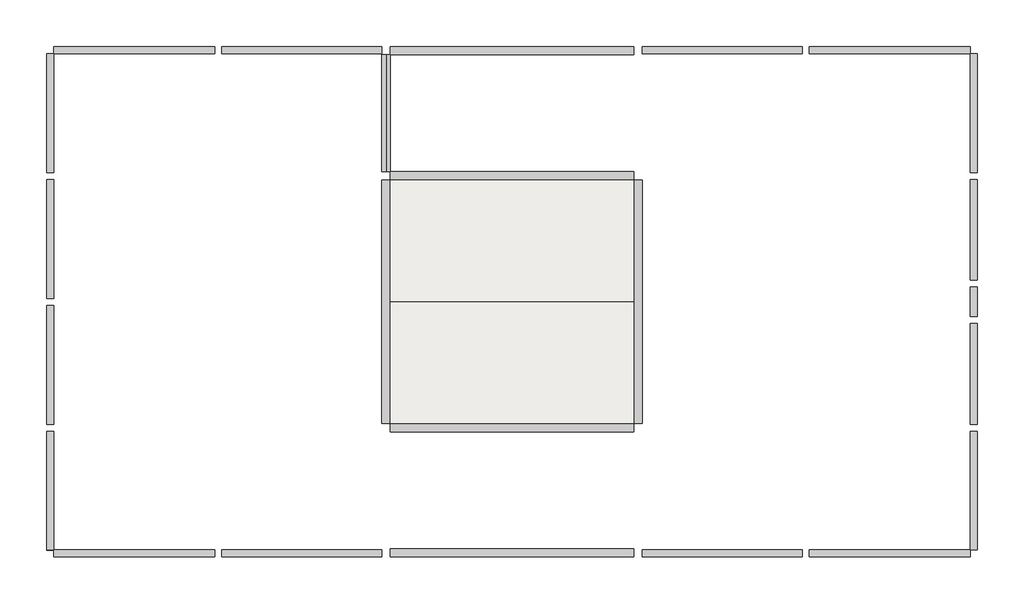
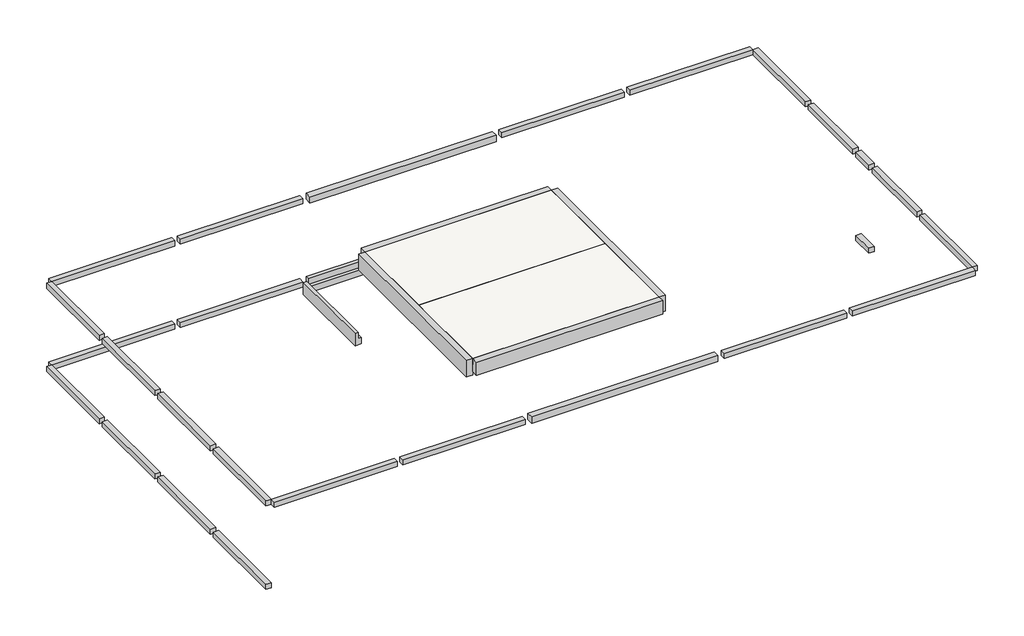
# One storey: 33 beams, 2 slabs.
"""IFC4 building model written with IfcOpenShell, lengths in millimetres."""

from ifc_helpers import new_model, si_unit, frame, origin, place, context, project, spatial, polyline, outline, extrude, faceted_brep, element, save

model = new_model("IFC4")

# Units and contexts
model_context = context("Model", 3, world=origin())
ifc_project = project(units=[si_unit("LENGTHUNIT", "METRE", prefix="MILLI")], contexts=[model_context])

# Site, building, storey
site = spatial("IfcSite", under=ifc_project)
building = spatial("IfcBuilding", under=site)
storey = spatial("IfcBuildingStorey", under=building, Name="E-CU02-AUXILIAR-Muro02", Elevation=6850.0)

# Beams
placement = place(None, origin())
element("IfcBeam", 1, ObjectType="E-VIGA-Hormigon : E-VIGA-Hormigon", at=placement, inside=storey, context=model_context, shape_type="Brep", body=[
    faceted_brep([(-21150.0, -13350.0, 6050.0), (-21150.0, -13350.0, 6850.0), (-21150.0, -4650.0, 6850.0), (-21150.0, -4650.0, 6050.0), (-20850.0, -13350.0, 6050.0), (-20850.0, -4650.0, 6050.0), (-20850.0, -8850.0, 6050.0), (-20850.0, -9150.0, 6050.0), (-20850.0, -13350.0, 6850.0), (-20850.0, -13350.0, 6550.0), (-20850.0, -4650.0, 6550.0), (-20850.0, -4650.0, 6850.0), (-20850.0, -9000.0, 6850.0)], [[[0, 1, 2, 3]], [[4, 0, 3, 5, 6, 7]], [[8, 9, 4, 7, 6, 5, 10, 11, 12]], [[1, 8, 12, 11, 2]], [[2, 11, 10, 5, 3]], [[1, 0, 4, 9, 8]]]),
])
element("IfcBeam", 2, ObjectType="E-VIGA-Hormigon : E-VIGA-Hormigon", at=placement, inside=storey, context=model_context, shape_type="Brep", body=[
    faceted_brep([(-12150.0, -13350.0, 6050.0), (-12150.0, -13350.0, 6550.0), (-12150.0, -13350.0, 6850.0), (-12150.0, -9000.0, 6850.0), (-12150.0, -4650.0, 6850.0), (-12150.0, -4650.0, 6550.0), (-12150.0, -4650.0, 6050.0), (-12150.0, -8850.0, 6050.0), (-12150.0, -9150.0, 6050.0), (-11850.0, -13350.0, 6050.0), (-11850.0, -4650.0, 6050.0), (-11850.0, -13350.0, 6850.0), (-11850.0, -4650.0, 6850.0)], [[[0, 1, 2, 3, 4, 5, 6, 7, 8]], [[9, 0, 8, 7, 6, 10]], [[11, 9, 10, 12]], [[2, 11, 12, 4, 3]], [[4, 12, 10, 6, 5]], [[2, 1, 0, 9, 11]]]),
])
element("IfcBeam", 3, ObjectType="E-VIGA-Hormigon : E-VIGA-Hormigon", at=placement, inside=storey, context=model_context, shape_type="Brep", body=[
    faceted_brep([(-12150.0, -4650.0, 6200.0), (-12150.0, -4650.0, 6550.0), (-12150.0, -4650.0, 6850.0), (-20850.0, -4650.0, 6850.0), (-20850.0, -4650.0, 6550.0), (-20850.0, -4650.0, 6200.0), (-12150.0, -4350.0, 6200.0), (-20850.0, -4350.0, 6200.0), (-12150.0, -4350.0, 6850.0), (-20850.0, -4350.0, 6850.0)], [[[0, 1, 2, 3, 4, 5]], [[6, 0, 5, 7]], [[8, 6, 7, 9]], [[2, 8, 9, 3]], [[3, 9, 7, 5, 4]], [[2, 1, 0, 6, 8]]]),
])
element("IfcBeam", 4, ObjectType="E-VIGA-Hormigon : E-VIGA-Hormigon", at=placement, inside=storey, context=model_context, shape_type="Brep", body=[
    faceted_brep([(-20850.0, -13650.0, 6850.0), (-20850.0, -13650.0, 6200.0), (-12150.0, -13650.0, 6200.0), (-12150.0, -13650.0, 6850.0), (-20850.0, -13350.0, 6200.0), (-12150.0, -13350.0, 6200.0), (-20850.0, -13350.0, 6550.0), (-20850.0, -13350.0, 6850.0), (-12150.0, -13350.0, 6850.0), (-12150.0, -13350.0, 6550.0)], [[[0, 1, 2, 3]], [[1, 4, 5, 2]], [[4, 6, 7, 8, 9, 5]], [[7, 0, 3, 8]], [[0, 7, 6, 4, 1]], [[3, 2, 5, 9, 8]]]),
])
element("IfcBeam", 5, ObjectType="E-VIGA-Hormigon : E-VIGA-Hormigon", at=placement, inside=storey, context=model_context, shape_type="Brep", body=[
    faceted_brep([(-20850.0, -9150.0, 6050.0), (-12150.0, -9150.0, 6050.0), (-12150.0, -9150.0, 6550.0), (-20850.0, -9150.0, 6550.0), (-20850.0, -8850.0, 6050.0), (-12150.0, -8850.0, 6050.0), (-20850.0, -8850.0, 6550.0), (-12150.0, -8850.0, 6550.0), (-20850.0, -9000.0, 6550.0), (-12150.0, -9000.0, 6550.0)], [[[0, 1, 2, 3]], [[0, 4, 5, 1]], [[5, 4, 6, 7]], [[4, 0, 3, 8, 6]], [[1, 5, 7, 9, 2]], [[7, 6, 8, 3, 2, 9]]]),
])
element("IfcBeam", 6, ObjectType="E-VIGA-Hormigon : E-VIGA-Hormigon", at=placement, inside=storey, context=model_context, shape_type="SweptSolid", body=[
    extrude(outline(polyline([(2730.0, -21150.0), (2130.0, -21150.0), (2130.0, -20850.0), (2430.0, -20850.0), (2430.0, -21000.0), (2730.0, -21000.0), (2730.0, -21150.0)])), frame((0.0, -4350.0, 0.0), z_axis=(0.0, 1.0, 0.0), x_axis=(0.0, 0.0, 1.0)), (0.0, 0.0, 1.0), 4175.0),
])
element("IfcBeam", 7, ObjectType="E-VIGA-Hormigon : E-VIGA-Hormigon", at=placement, inside=storey, context=model_context, shape_type="SweptSolid", body=[
    extrude(outline(polyline([(125.0, 2730.0), (125.0, 2130.0), (-175.0, 2130.0), (-175.0, 2430.0), (-25.0, 2430.0), (-25.0, 2730.0), (125.0, 2730.0)])), frame((-20850.0, 0.0, 0.0), z_axis=(1.0, 0.0, 0.0), x_axis=(0.0, 1.0, 0.0)), (0.0, 0.0, 1.0), 8700.0),
])
element("IfcBeam", 8, ObjectType="E-VIGA-Hormigon : E-VIGA-Hormigon", at=placement, inside=storey, context=model_context, shape_type="SweptSolid", body=[
    extrude(outline(polyline([(-33125.0, -13625.0), (-32875.0, -13625.0), (-32875.0, -17875.0), (-33125.0, -17875.0), (-33125.0, -13625.0)])), frame((0.0, 0.0, 2480.0), z_axis=(0.0, 0.0, 1.0), x_axis=(1.0, 0.0, 0.0)), (0.0, 0.0, 1.0), 250.0),
])
element("IfcBeam", 9, ObjectType="E-VIGA-Hormigon : E-VIGA-Hormigon", at=placement, inside=storey, context=model_context, shape_type="SweptSolid", body=[
    extrude(outline(polyline([(-33125.0, -9125.0), (-32875.0, -9125.0), (-32875.0, -13375.0), (-33125.0, -13375.0), (-33125.0, -9125.0)])), frame((0.0, 0.0, 2480.0), z_axis=(0.0, 0.0, 1.0), x_axis=(1.0, 0.0, 0.0)), (0.0, 0.0, 1.0), 250.0),
])
element("IfcBeam", 10, ObjectType="E-VIGA-Hormigon : E-VIGA-Hormigon", at=placement, inside=storey, context=model_context, shape_type="SweptSolid", body=[
    extrude(outline(polyline([(-33125.0, -4625.0), (-32875.0, -4625.0), (-32875.0, -8875.0), (-33125.0, -8875.0), (-33125.0, -4625.0)])), frame((0.0, 0.0, 2480.0), z_axis=(0.0, 0.0, 1.0), x_axis=(1.0, 0.0, 0.0)), (0.0, 0.0, 1.0), 250.0),
])
element("IfcBeam", 11, ObjectType="E-VIGA-Hormigon : E-VIGA-Hormigon", at=placement, inside=storey, context=model_context, shape_type="SweptSolid", body=[
    extrude(outline(polyline([(-33125.0, -125.0), (-32875.0, -125.0), (-32875.0, -4375.0), (-33125.0, -4375.0), (-33125.0, -125.0)])), frame((0.0, 0.0, 2480.0), z_axis=(0.0, 0.0, 1.0), x_axis=(1.0, 0.0, 0.0)), (0.0, 0.0, 1.0), 250.0),
])
element("IfcBeam", 12, ObjectType="E-VIGA-Hormigon : E-VIGA-Hormigon", at=placement, inside=storey, context=model_context, shape_type="SweptSolid", body=[
    extrude(outline(polyline([(-125.0, -8475.0), (125.0, -8475.0), (125.0, -9525.0), (-125.0, -9525.0), (-125.0, -8475.0)])), frame((0.0, 0.0, 2480.0), z_axis=(0.0, 0.0, 1.0), x_axis=(1.0, 0.0, 0.0)), (0.0, 0.0, 1.0), 250.0),
])
element("IfcBeam", 13, ObjectType="E-VIGA-Hormigon : E-VIGA-Hormigon", at=placement, inside=storey, context=model_context, shape_type="SweptSolid", body=[
    extrude(outline(polyline([(-33125.0, -13625.0), (-32875.0, -13625.0), (-32875.0, -17875.0), (-33125.0, -17875.0), (-33125.0, -13625.0)])), frame((0.0, 0.0, 6600.0), z_axis=(0.0, 0.0, 1.0), x_axis=(1.0, 0.0, 0.0)), (0.0, 0.0, 1.0), 250.0),
])
element("IfcBeam", 14, ObjectType="E-VIGA-Hormigon : E-VIGA-Hormigon", at=placement, inside=storey, context=model_context, shape_type="SweptSolid", body=[
    extrude(outline(polyline([(-33125.0, -9125.0), (-32875.0, -9125.0), (-32875.0, -13375.0), (-33125.0, -13375.0), (-33125.0, -9125.0)])), frame((0.0, 0.0, 6600.0), z_axis=(0.0, 0.0, 1.0), x_axis=(1.0, 0.0, 0.0)), (0.0, 0.0, 1.0), 250.0),
])
element("IfcBeam", 15, ObjectType="E-VIGA-Hormigon : E-VIGA-Hormigon", at=placement, inside=storey, context=model_context, shape_type="SweptSolid", body=[
    extrude(outline(polyline([(-33125.0, -4625.0), (-32875.0, -4625.0), (-32875.0, -8875.0), (-33125.0, -8875.0), (-33125.0, -4625.0)])), frame((0.0, 0.0, 6600.0), z_axis=(0.0, 0.0, 1.0), x_axis=(1.0, 0.0, 0.0)), (0.0, 0.0, 1.0), 250.0),
])
element("IfcBeam", 16, ObjectType="E-VIGA-Hormigon : E-VIGA-Hormigon", at=placement, inside=storey, context=model_context, shape_type="SweptSolid", body=[
    extrude(outline(polyline([(-33125.0, -125.0), (-32875.0, -125.0), (-32875.0, -4375.0), (-33125.0, -4375.0), (-33125.0, -125.0)])), frame((0.0, 0.0, 6600.0), z_axis=(0.0, 0.0, 1.0), x_axis=(1.0, 0.0, 0.0)), (0.0, 0.0, 1.0), 250.0),
])
element("IfcBeam", 17, ObjectType="E-VIGA-Hormigon : E-VIGA-Hormigon", at=placement, inside=storey, context=model_context, shape_type="SweptSolid", body=[
    extrude(outline(polyline([(125.0, -13625.0), (125.0, -17875.0), (-125.0, -17875.0), (-125.0, -13625.0), (125.0, -13625.0)])), frame((0.0, 0.0, 6600.0), z_axis=(0.0, 0.0, 1.0), x_axis=(1.0, 0.0, 0.0)), (0.0, 0.0, 1.0), 250.0),
])
element("IfcBeam", 18, ObjectType="E-VIGA-Hormigon : E-VIGA-Hormigon", at=placement, inside=storey, context=model_context, shape_type="SweptSolid", body=[
    extrude(outline(polyline([(125.0, -13375.0), (-125.0, -13375.0), (-125.0, -9775.0), (125.0, -9775.0), (125.0, -13375.0)])), frame((0.0, 0.0, 6600.0), z_axis=(0.0, 0.0, 1.0), x_axis=(1.0, 0.0, 0.0)), (0.0, 0.0, 1.0), 250.0),
])
element("IfcBeam", 19, ObjectType="E-VIGA-Hormigon : E-VIGA-Hormigon", at=placement, inside=storey, context=model_context, shape_type="SweptSolid", body=[
    extrude(outline(polyline([(-125.0, -4625.0), (125.0, -4625.0), (125.0, -8225.0), (-125.0, -8225.0), (-125.0, -4625.0)])), frame((0.0, 0.0, 6600.0), z_axis=(0.0, 0.0, 1.0), x_axis=(1.0, 0.0, 0.0)), (0.0, 0.0, 1.0), 250.0),
])
element("IfcBeam", 20, ObjectType="E-VIGA-Hormigon : E-VIGA-Hormigon", at=placement, inside=storey, context=model_context, shape_type="SweptSolid", body=[
    extrude(outline(polyline([(125.0, -125.0), (125.0, -4375.0), (-125.0, -4375.0), (-125.0, -125.0), (125.0, -125.0)])), frame((0.0, 0.0, 6600.0), z_axis=(0.0, 0.0, 1.0), x_axis=(1.0, 0.0, 0.0)), (0.0, 0.0, 1.0), 250.0),
])
element("IfcBeam", 21, ObjectType="E-VIGA-Hormigon : E-VIGA-Hormigon", at=placement, inside=storey, context=model_context, shape_type="SweptSolid", body=[
    extrude(outline(polyline([(-27125.0, 125.0), (-27125.0, -125.0), (-32875.0, -125.0), (-32875.0, 125.0), (-27125.0, 125.0)])), frame((0.0, 0.0, 2480.0), z_axis=(0.0, 0.0, 1.0), x_axis=(1.0, 0.0, 0.0)), (0.0, 0.0, 1.0), 250.0),
])
element("IfcBeam", 22, ObjectType="E-VIGA-Hormigon : E-VIGA-Hormigon", at=placement, inside=storey, context=model_context, shape_type="SweptSolid", body=[
    extrude(outline(polyline([(-26875.0, -125.0), (-26875.0, 125.0), (-21150.0, 125.0), (-21150.0, -125.0), (-26875.0, -125.0)])), frame((0.0, 0.0, 2480.0), z_axis=(0.0, 0.0, 1.0), x_axis=(1.0, 0.0, 0.0)), (0.0, 0.0, 1.0), 250.0),
])
element("IfcBeam", 23, ObjectType="E-VIGA-Hormigon : E-VIGA-Hormigon", at=placement, inside=storey, context=model_context, shape_type="SweptSolid", body=[
    extrude(outline(polyline([(-125.0, -8475.0), (125.0, -8475.0), (125.0, -9525.0), (-125.0, -9525.0), (-125.0, -8475.0)])), frame((0.0, 0.0, 6600.0), z_axis=(0.0, 0.0, 1.0), x_axis=(1.0, 0.0, 0.0)), (0.0, 0.0, 1.0), 250.0),
])
element("IfcBeam", 24, ObjectType="E-VIGA-Hormigon : E-VIGA-Hormigon", at=placement, inside=storey, context=model_context, shape_type="SweptSolid", body=[
    extrude(outline(polyline([(-27125.0, 125.0), (-27125.0, -125.0), (-32875.0, -125.0), (-32875.0, 125.0), (-27125.0, 125.0)])), frame((0.0, 0.0, 6600.0), z_axis=(0.0, 0.0, 1.0), x_axis=(1.0, 0.0, 0.0)), (0.0, 0.0, 1.0), 250.0),
])
element("IfcBeam", 25, ObjectType="E-VIGA-Hormigon : E-VIGA-Hormigon", at=placement, inside=storey, context=model_context, shape_type="SweptSolid", body=[
    extrude(outline(polyline([(-26875.0, -125.0), (-26875.0, 125.0), (-21150.0, 125.0), (-21150.0, -125.0), (-26875.0, -125.0)])), frame((0.0, 0.0, 6600.0), z_axis=(0.0, 0.0, 1.0), x_axis=(1.0, 0.0, 0.0)), (0.0, 0.0, 1.0), 250.0),
])
element("IfcBeam", 26, ObjectType="E-VIGA-Hormigon : E-VIGA-Hormigon", at=placement, inside=storey, context=model_context, shape_type="SweptSolid", body=[
    extrude(outline(polyline([(-12150.0, 125.0), (-12150.0, -175.0), (-20850.0, -175.0), (-20850.0, 125.0), (-12150.0, 125.0)])), frame((0.0, 0.0, 6550.0), z_axis=(0.0, 0.0, 1.0), x_axis=(1.0, 0.0, 0.0)), (0.0, 0.0, 1.0), 300.0),
])
element("IfcBeam", 27, ObjectType="E-VIGA-Hormigon : E-VIGA-Hormigon", at=placement, inside=storey, context=model_context, shape_type="SweptSolid", body=[
    extrude(outline(polyline([(-5875.0, 125.0), (-125.0, 125.0), (-125.0, -125.0), (-5875.0, -125.0), (-5875.0, 125.0)])), frame((0.0, 0.0, 6600.0), z_axis=(0.0, 0.0, 1.0), x_axis=(1.0, 0.0, 0.0)), (0.0, 0.0, 1.0), 250.0),
])
element("IfcBeam", 28, ObjectType="E-VIGA-Hormigon : E-VIGA-Hormigon", at=placement, inside=storey, context=model_context, shape_type="SweptSolid", body=[
    extrude(outline(polyline([(-6125.0, 125.0), (-6125.0, -125.0), (-11850.0, -125.0), (-11850.0, 125.0), (-6125.0, 125.0)])), frame((0.0, 0.0, 6600.0), z_axis=(0.0, 0.0, 1.0), x_axis=(1.0, 0.0, 0.0)), (0.0, 0.0, 1.0), 250.0),
])
element("IfcBeam", 29, ObjectType="E-VIGA-Hormigon : E-VIGA-Hormigon", at=placement, inside=storey, context=model_context, shape_type="SweptSolid", body=[
    extrude(outline(polyline([(-27125.0, -17875.0), (-27125.0, -18125.0), (-32875.0, -18125.0), (-32875.0, -17875.0), (-27125.0, -17875.0)])), frame((0.0, 0.0, 6600.0), z_axis=(0.0, 0.0, 1.0), x_axis=(1.0, 0.0, 0.0)), (0.0, 0.0, 1.0), 250.0),
])
element("IfcBeam", 30, ObjectType="E-VIGA-Hormigon : E-VIGA-Hormigon", at=placement, inside=storey, context=model_context, shape_type="SweptSolid", body=[
    extrude(outline(polyline([(-26875.0, -18125.0), (-26875.0, -17875.0), (-21150.0, -17875.0), (-21150.0, -18125.0), (-26875.0, -18125.0)])), frame((0.0, 0.0, 6600.0), z_axis=(0.0, 0.0, 1.0), x_axis=(1.0, 0.0, 0.0)), (0.0, 0.0, 1.0), 250.0),
])
element("IfcBeam", 31, ObjectType="E-VIGA-Hormigon : E-VIGA-Hormigon", at=placement, inside=storey, context=model_context, shape_type="SweptSolid", body=[
    extrude(outline(polyline([(-5875.0, -17875.0), (-125.0, -17875.0), (-125.0, -18125.0), (-5875.0, -18125.0), (-5875.0, -17875.0)])), frame((0.0, 0.0, 6600.0), z_axis=(0.0, 0.0, 1.0), x_axis=(1.0, 0.0, 0.0)), (0.0, 0.0, 1.0), 250.0),
])
element("IfcBeam", 32, ObjectType="E-VIGA-Hormigon : E-VIGA-Hormigon", at=placement, inside=storey, context=model_context, shape_type="SweptSolid", body=[
    extrude(outline(polyline([(-6125.0, -17875.0), (-6125.0, -18125.0), (-11850.0, -18125.0), (-11850.0, -17875.0), (-6125.0, -17875.0)])), frame((0.0, 0.0, 6600.0), z_axis=(0.0, 0.0, 1.0), x_axis=(1.0, 0.0, 0.0)), (0.0, 0.0, 1.0), 250.0),
])
element("IfcBeam", 33, ObjectType="E-VIGA-Hormigon : E-VIGA-Hormigon", at=placement, inside=storey, context=model_context, shape_type="SweptSolid", body=[
    extrude(outline(polyline([(-12150.0, -17825.0), (-12150.0, -18125.0), (-20850.0, -18125.0), (-20850.0, -17825.0), (-12150.0, -17825.0)])), frame((0.0, 0.0, 6550.0), z_axis=(0.0, 0.0, 1.0), x_axis=(1.0, 0.0, 0.0)), (0.0, 0.0, 1.0), 300.0),
])

# Slabs
element("IfcSlab", 34, ObjectType="FORJADO 2_PABLO", at=placement, inside=storey, context=model_context, shape_type="Brep", body=[
    faceted_brep([(-12150.0, -4650.0, 6550.0), (-12150.0, -8850.0, 6550.0), (-12150.0, -9000.0, 6550.0), (-20850.0, -9000.0, 6550.0), (-20850.0, -8850.0, 6550.0), (-20850.0, -4650.0, 6550.0), (-12150.0, -9000.0, 6850.0), (-12150.0, -4650.0, 6850.0), (-20850.0, -4650.0, 6850.0), (-20850.0, -9000.0, 6850.0)], [[[0, 1, 2, 3, 4, 5]], [[6, 7, 8, 9]], [[2, 6, 9, 3]], [[2, 1, 0, 7, 6]], [[0, 5, 8, 7]], [[5, 4, 3, 9, 8]]]),
])
element("IfcSlab", 35, ObjectType="FORJADO 1_PABLO", at=placement, inside=storey, context=model_context, shape_type="Brep", body=[
    faceted_brep([(-12150.0, -9000.0, 6550.0), (-12150.0, -9150.0, 6550.0), (-12150.0, -13350.0, 6550.0), (-20850.0, -13350.0, 6550.0), (-20850.0, -9150.0, 6550.0), (-20850.0, -9000.0, 6550.0), (-12150.0, -13350.0, 6850.0), (-12150.0, -9000.0, 6850.0), (-20850.0, -9000.0, 6850.0), (-20850.0, -13350.0, 6850.0)], [[[0, 1, 2, 3, 4, 5]], [[6, 7, 8, 9]], [[7, 0, 5, 8]], [[2, 1, 0, 7, 6]], [[5, 4, 3, 9, 8]], [[3, 2, 6, 9]]]),
])

save(model, "model.ifc")

# Revit data of these elements
# Type "E-VIGA-Hormigon : E-VIGA-Hormigon"
#   Numeration [instance default] = ""
#   Length [instance default] = 3.000 m
#   AnchoViga [instance default] = 0.200 m
#   AltoViga [instance default] = 0.300 m
# Type "FORJADO 2_PABLO"
#   Function = 0
#   Layers, outside or top first: 0.140 m "Hormigón, moldeado in situ" (function 1); 0.160 m "Ladrillo, hueco" (function 1)
# Type "FORJADO 1_PABLO"
#   Function = 0
#   Layers, outside or top first: 0.140 m "Hormigón, moldeado in situ" (function 1); 0.160 m "Forjado vigueta semirresistente y bovedilla cerámica" (function 1)
# Elements 1, 2, 5 (IfcBeam, "E-VIGA-Hormigon : E-VIGA-Hormigon")
#   Comments = ""
#   Numeration = ""
#   AnchoViga = 0.300 m
#   AltoViga = 0.800 m
#   Phase Created = Nueva construcción
#   Materials on its faces: "Concrete, Cast-in-Place, Gray"
# Elements 3, 4 (IfcBeam, "E-VIGA-Hormigon : E-VIGA-Hormigon")
#   Comments = ""
#   Numeration = ""
#   AnchoViga = 0.300 m
#   AltoViga = 0.650 m
#   Phase Created = Nueva construcción
#   Materials on its faces: "Concrete, Cast-in-Place, Gray"
# Elements 6, 7 (IfcBeam, "E-VIGA-Hormigon : E-VIGA-Hormigon")
#   Comments = ""
#   Numeration = ""
#   AnchoViga = 0.300 m
#   AltoViga = 0.600 m
#   Phase Created = Nueva construcción
#   Materials on its faces: "Concrete, Cast-in-Place, Gray"
# Elements 8, 9, 10, 11, 12, 13, 14, 15, 16, 17, 18, 19, 20, 21, 22, 23, 24, 25, 27, 28, 29, 30, 31, 32 (IfcBeam, "E-VIGA-Hormigon : E-VIGA-Hormigon")
#   Comments = ""
#   Numeration = ""
#   AnchoViga = 0.250 m
#   AltoViga = 0.250 m
#   Phase Created = Nueva construcción
#   Materials on its faces: "Concrete, Cast-in-Place, Gray"
# Elements 26, 33 (IfcBeam, "E-VIGA-Hormigon : E-VIGA-Hormigon")
#   Comments = ""
#   Numeration = ""
#   AnchoViga = 0.300 m
#   AltoViga = 0.300 m
#   Phase Created = Nueva construcción
#   Materials on its faces: "Concrete, Cast-in-Place, Gray"
# Element 34 (IfcSlab, "FORJADO 2_PABLO")
#   Comments = ""
#   Height Offset From Level = 0.000 m
#   built-in parameter 1001954 = 1
#   Phase Created = Nueva construcción
#   Materials on its faces: "Ladrillo, hueco", "Hormigón, moldeado in situ"
# Element 35 (IfcSlab, "FORJADO 1_PABLO")
#   Height Offset From Level = 0.000 m
#   built-in parameter 1001954 = 1
#   Phase Created = Nueva construcción
#   Materials on its faces: "Forjado vigueta semirresistente y bovedilla cerámica", "Hormigón, moldeado in situ"
# Materials
#   "Hormigón, moldeado in situ": class "Hormigón", colour RGB 192 192 192, transparency 0, Description = "material físico", Cost = 0
#   "Ladrillo, hueco": class "Albañilería", colour RGB 120 120 120, transparency 0, Description = "Ladrillo hueco", Cost = 0
#   "Forjado vigueta semirresistente y bovedilla cerámica": class "Albañilería", colour RGB 120 120 120, transparency 0, Description = "Ladrillo hueco", Cost = 0
#   "Concrete, Cast-in-Place, Gray": class "Concrete", colour RGB 129 132 118, transparency 0, Description = "Cast-in-place concrete", Cost = 0
